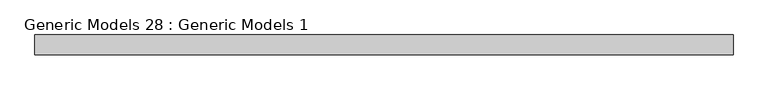
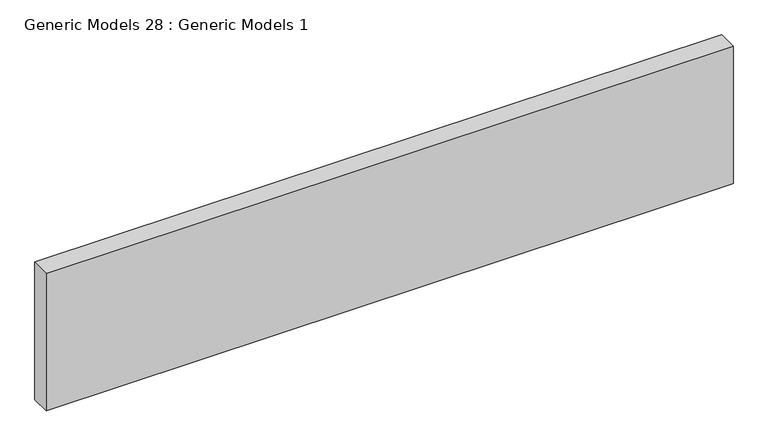
"""IFC4 building model written with IfcOpenShell, lengths in millimetres: proxy geometry, Generic Models 28 : Generic Models 1."""

from ifc_helpers import new_model, si_unit, frame, origin, place, context, project, spatial, polyline, outline, extrude, source, transform, mapped, element, save


def generic_models_28_generic_models_1_2f61f013(model_context):
    return source(origin(), model_context, "Body", "SweptSolid", [
        extrude(outline(polyline([(-9255.2986296, 8371.4650592), (-9255.2986296, 8409.5650592), (-7909.0986296, 8409.5650592), (-7909.0986296, 8371.4650592), (-9255.2986296, 8371.4650592)])), frame((0.0, 0.0, 126485.396), z_axis=(0.0, 0.0, 1.0), x_axis=(1.0, 0.0, 0.0)), (0.0, 0.0, 1.0), 285.75),
    ])


if __name__ == "__main__":
    model = new_model("IFC4")
    model_context = context("Model", 3, world=origin())
    ifc_project = project(units=[si_unit("LENGTHUNIT", "METRE", prefix="MILLI")], contexts=[model_context])
    site = spatial("IfcSite", under=ifc_project)
    building = spatial("IfcBuilding", under=site)
    placement = place(None, origin())
    generic_models_28_generic_models_1_shape = generic_models_28_generic_models_1_2f61f013(model_context)
    element("IfcBuildingElementProxy", 1, Name="Generic Models 28 : Generic Models 1", ObjectType="Generic Models 28 : Generic Models 1", at=placement, inside=building, context=model_context, shape_type="MappedRepresentation", body=[
        mapped(generic_models_28_generic_models_1_shape, transform((0.0, 0.0, 0.0), x_axis=(1.0, 0.0, 0.0), y_axis=(0.0, 1.0, 0.0), z_axis=(0.0, 0.0, 1.0))),
    ])
    save(model, "model.ifc")

# Revit data of these elements
# Element 1 (IfcBuildingElementProxy, "Generic Models 28 : Generic Models 1")
#   Materials on its faces: "_STRUCTURAL MEMBER (SEE STRUCT. DWGS)"
# Materials
#   "_STRUCTURAL MEMBER (SEE STRUCT. DWGS)": class "Generic", colour RGB 209 182 141, transparency 0, Cost = 0
